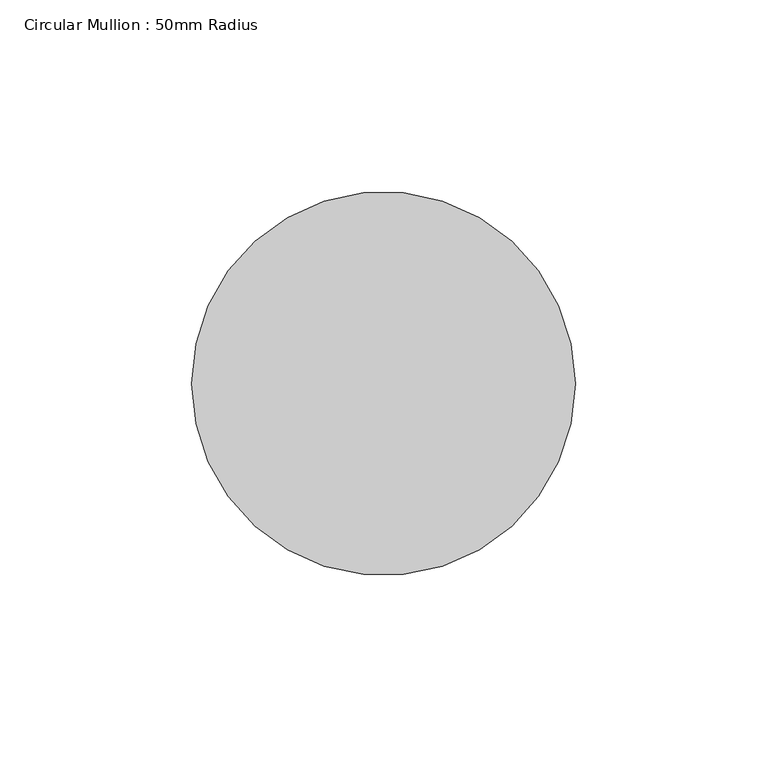
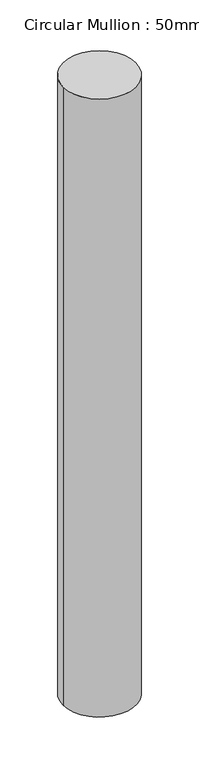
"""IFC4 building model written with IfcOpenShell, lengths in millimetres: member geometry, Circular Mullion : 50mm Radius."""

from ifc_helpers import new_model, si_unit, point, frame, origin, origin_2d, place, context, project, spatial, circle_curve, trimmed, segment, composite_curve, outline, extrude, source, transform, mapped, element, save


def circular_mullion_50mm_radius_d812c722(model_context):
    return source(origin(), model_context, "Body", "SweptSolid", [
        extrude(outline(composite_curve([segment(trimmed(circle_curve(origin_2d(), 50.0), [point((50.0, 0.0))], [point((-50.0, 0.0))], False, "CARTESIAN"), True, "CONTINUOUS"), segment(trimmed(circle_curve(origin_2d(), 50.0), [point((-50.0, 0.0))], [point((50.0, 0.0))], False, "CARTESIAN"), True, "CONTINUOUS")], self_intersect=False)), frame((0.0, 0.0, -897.5372577), z_axis=(0.0, 0.0, 1.0), x_axis=(1.0, 0.0, 0.0)), (0.0, 0.0, 1.0), 897.5372577),
    ])


if __name__ == "__main__":
    model = new_model("IFC4")
    model_context = context("Model", 3, world=origin())
    ifc_project = project(units=[si_unit("LENGTHUNIT", "METRE", prefix="MILLI")], contexts=[model_context])
    site = spatial("IfcSite", under=ifc_project)
    building = spatial("IfcBuilding", under=site)
    placement = place(None, origin())
    circular_mullion_50mm_radius_shape = circular_mullion_50mm_radius_d812c722(model_context)
    element("IfcMember", 1, ObjectType="Circular Mullion : 50mm Radius", at=placement, inside=building, context=model_context, shape_type="MappedRepresentation", body=[
        mapped(circular_mullion_50mm_radius_shape, transform((0.0, 0.0, 0.0), x_axis=(1.0, 0.0, 0.0), y_axis=(0.0, 1.0, 0.0), z_axis=(0.0, 0.0, 1.0))),
    ])
    save(model, "model.ifc")

# Revit data of these elements
# Type "Circular Mullion : 50mm Radius"
#   built-in parameter 1007350 = 0.164042 (stored number, unit not read)
# Element 1 (IfcMember, "Circular Mullion : 50mm Radius")
#   Materials on its faces: "Aluminium"
# Materials
#   "Aluminium": class "Metal", colour RGB 247 247 247, transparency 0, Description = "Aluminium 6061", Cost = 0
